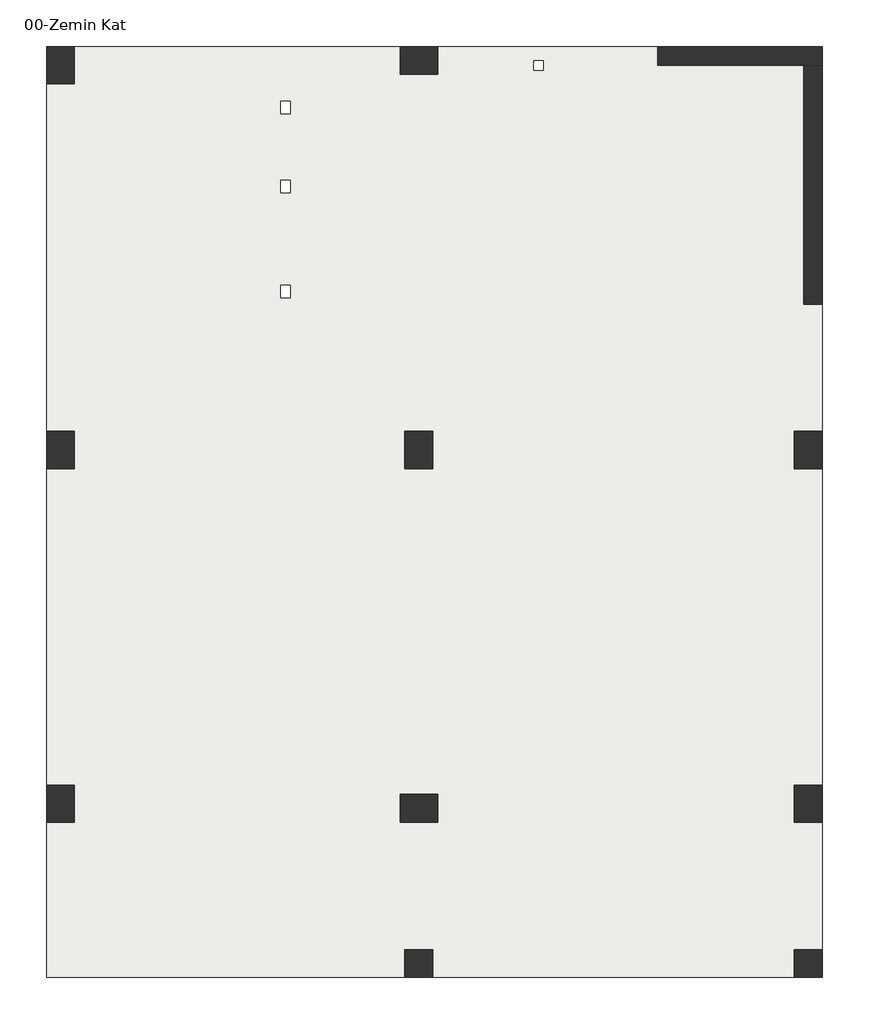
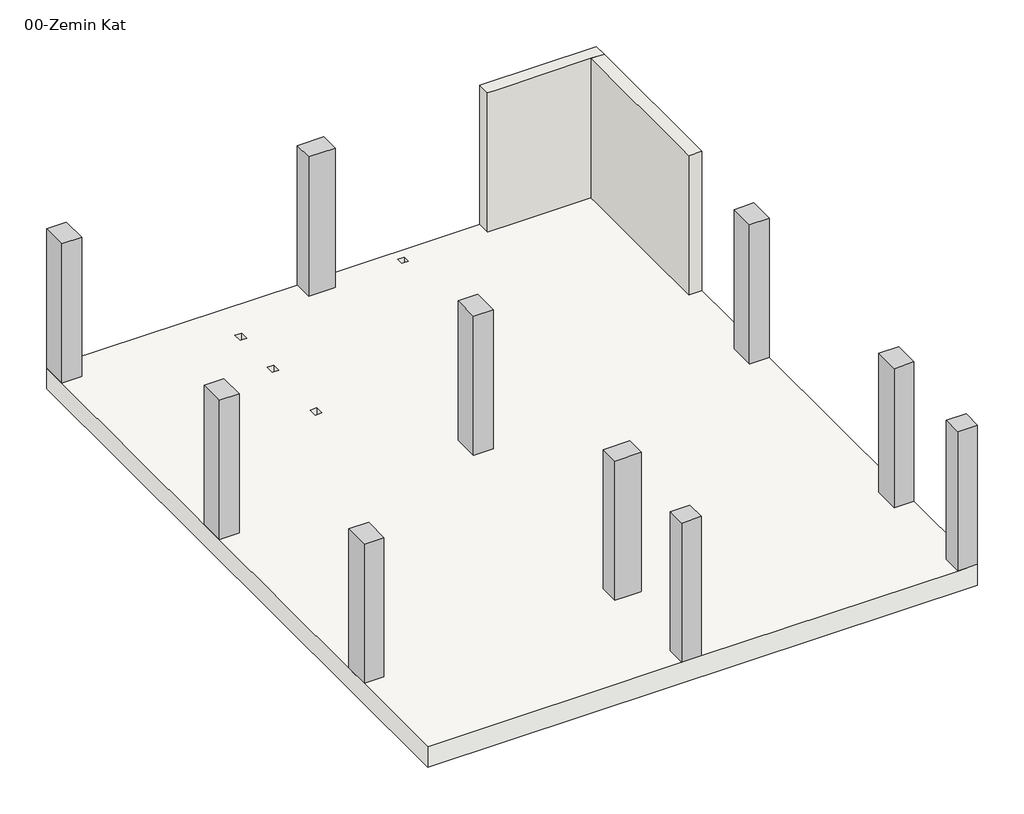
# One storey: 10 columns, 2 walls, 1 slab.
"""IFC4 building model written with IfcOpenShell, lengths in millimetres."""

from ifc_helpers import new_model, si_unit, frame, origin, place, context, project, spatial, polyline, outline, extrude, faceted_brep, element, save

model = new_model("IFC4")

# Units and contexts
model_context = context("Model", 3, world=origin())
ifc_project = project(units=[si_unit("LENGTHUNIT", "METRE", prefix="MILLI")], contexts=[model_context])

# Site, building, storey
site = spatial("IfcSite", under=ifc_project)
building = spatial("IfcBuilding", under=site)
storey = spatial("IfcBuildingStorey", under=building, Name="00-Zemin Kat", Elevation=93780.0)

# Columns
placement = place(None, origin())
element("IfcColumn", 1, ObjectType="M_Concrete-Rectangular-Column : 45x60cm Kolon", at=placement, inside=storey, context=model_context, shape_type="SweptSolid", body=[
    extrude(outline(polyline([(450.0, 15000.0), (450.0, 14400.0), (0.0, 14400.0), (0.0, 15000.0), (450.0, 15000.0)])), frame((0.0, 0.0, 93780.0), z_axis=(0.0, 0.0, 1.0), x_axis=(1.0, 0.0, 0.0)), (0.0, 0.0, 1.0), 3350.0),
])
element("IfcColumn", 2, ObjectType="M_Concrete-Rectangular-Column : 45x60cm Kolon", at=placement, inside=storey, context=model_context, shape_type="SweptSolid", body=[
    extrude(outline(polyline([(450.0, 8800.0), (450.0, 8200.0), (0.0, 8200.0), (0.0, 8800.0), (450.0, 8800.0)])), frame((0.0, 0.0, 93780.0), z_axis=(0.0, 0.0, 1.0), x_axis=(1.0, 0.0, 0.0)), (0.0, 0.0, 1.0), 3350.0),
])
element("IfcColumn", 3, ObjectType="M_Concrete-Rectangular-Column : 45x60cm Kolon", at=placement, inside=storey, context=model_context, shape_type="SweptSolid", body=[
    extrude(outline(polyline([(450.0, 3100.0), (450.0, 2500.0), (0.0, 2500.0), (0.0, 3100.0), (450.0, 3100.0)])), frame((0.0, 0.0, 93780.0), z_axis=(0.0, 0.0, 1.0), x_axis=(1.0, 0.0, 0.0)), (0.0, 0.0, 1.0), 3350.0),
])
element("IfcColumn", 4, ObjectType="M_Concrete-Rectangular-Column : 45x60cm Kolon", at=placement, inside=storey, context=model_context, shape_type="SweptSolid", body=[
    extrude(outline(polyline([(6225.0, 8800.0), (6225.0, 8200.0), (5775.0, 8200.0), (5775.0, 8800.0), (6225.0, 8800.0)])), frame((0.0, 0.0, 93780.0), z_axis=(0.0, 0.0, 1.0), x_axis=(1.0, 0.0, 0.0)), (0.0, 0.0, 1.0), 3350.0),
])
element("IfcColumn", 5, ObjectType="M_Concrete-Rectangular-Column : 45x60cm Kolon", at=placement, inside=storey, context=model_context, shape_type="SweptSolid", body=[
    extrude(outline(polyline([(12500.0, 8800.0), (12500.0, 8200.0), (12050.0, 8200.0), (12050.0, 8800.0), (12500.0, 8800.0)])), frame((0.0, 0.0, 93780.0), z_axis=(0.0, 0.0, 1.0), x_axis=(1.0, 0.0, 0.0)), (0.0, 0.0, 1.0), 3350.0),
])
element("IfcColumn", 6, ObjectType="M_Concrete-Rectangular-Column : 45x60cm Kolon", at=placement, inside=storey, context=model_context, shape_type="SweptSolid", body=[
    extrude(outline(polyline([(12500.0, 3100.0), (12500.0, 2500.0), (12050.0, 2500.0), (12050.0, 3100.0), (12500.0, 3100.0)])), frame((0.0, 0.0, 93780.0), z_axis=(0.0, 0.0, 1.0), x_axis=(1.0, 0.0, 0.0)), (0.0, 0.0, 1.0), 3350.0),
])
element("IfcColumn", 7, ObjectType="M_Concrete-Rectangular-Column : 45x60cm Kolon", at=placement, inside=storey, context=model_context, shape_type="SweptSolid", body=[
    extrude(outline(polyline([(5700.0, 15000.0), (6300.0, 15000.0), (6300.0, 14550.0), (5700.0, 14550.0), (5700.0, 15000.0)])), frame((0.0, 0.0, 93780.0), z_axis=(0.0, 0.0, 1.0), x_axis=(1.0, 0.0, 0.0)), (0.0, 0.0, 1.0), 3350.0),
])
element("IfcColumn", 8, ObjectType="M_Concrete-Rectangular-Column : 45x45cm Kolon", at=placement, inside=storey, context=model_context, shape_type="SweptSolid", body=[
    extrude(outline(polyline([(6225.0, 450.0), (6225.0, 0.0), (5775.0, 0.0), (5775.0, 450.0), (6225.0, 450.0)])), frame((0.0, 0.0, 93780.0), z_axis=(0.0, 0.0, 1.0), x_axis=(1.0, 0.0, 0.0)), (0.0, 0.0, 1.0), 3350.0),
])
element("IfcColumn", 9, ObjectType="M_Concrete-Rectangular-Column : 45x60cm Kolon", at=placement, inside=storey, context=model_context, shape_type="SweptSolid", body=[
    extrude(outline(polyline([(5700.0, 2950.0), (6300.0, 2950.0), (6300.0, 2500.0), (5700.0, 2500.0), (5700.0, 2950.0)])), frame((0.0, 0.0, 93780.0), z_axis=(0.0, 0.0, 1.0), x_axis=(1.0, 0.0, 0.0)), (0.0, 0.0, 1.0), 3350.0),
])
element("IfcColumn", 10, ObjectType="M_Concrete-Rectangular-Column : 45x45cm Kolon", at=placement, inside=storey, context=model_context, shape_type="SweptSolid", body=[
    extrude(outline(polyline([(12500.0, 450.0), (12500.0, 0.0), (12050.0, 0.0), (12050.0, 450.0), (12500.0, 450.0)])), frame((0.0, 0.0, 93780.0), z_axis=(0.0, 0.0, 1.0), x_axis=(1.0, 0.0, 0.0)), (0.0, 0.0, 1.0), 3350.0),
])

# Slab
element("IfcSlab", 11, ObjectType="50 cm döşeme", at=placement, inside=storey, context=model_context, shape_type="Brep", body=[
    faceted_brep([(12500.0, 15000.0, 93280.0), (12500.0, 0.0, 93280.0), (0.0, 0.0, 93280.0), (0.0, 15000.0, 93280.0), (3925.0, 14120.0, 93280.0), (3775.0, 14120.0, 93280.0), (3775.0, 13920.0, 93280.0), (3925.0, 13920.0, 93280.0), (3925.0, 12846.5789726, 93280.0), (3775.0, 12846.5789726, 93280.0), (3775.0, 12646.5789726, 93280.0), (3925.0, 12646.5789726, 93280.0), (3925.0, 11154.975, 93280.0), (3775.0, 11154.975, 93280.0), (3775.0, 10954.975, 93280.0), (3925.0, 10954.975, 93280.0), (7852.5, 14620.0, 93280.0), (8002.5, 14620.0, 93280.0), (8002.5, 14770.0, 93280.0), (7852.5, 14770.0, 93280.0), (12500.0, 15000.0, 93780.0), (6300.0, 15000.0, 93780.0), (5700.0, 15000.0, 93780.0), (450.0, 15000.0, 93780.0), (0.0, 15000.0, 93780.0), (0.0, 14400.0, 93780.0), (0.0, 8800.0, 93780.0), (0.0, 8200.0, 93780.0), (0.0, 3100.0, 93780.0), (0.0, 2500.0, 93780.0), (0.0, 0.0, 93780.0), (5775.0, 0.0, 93780.0), (6225.0, 0.0, 93780.0), (12050.0, 0.0, 93780.0), (12500.0, 0.0, 93780.0), (12500.0, 450.0, 93780.0), (12500.0, 2500.0, 93780.0), (12500.0, 3100.0, 93780.0), (12500.0, 8200.0, 93780.0), (12500.0, 8800.0, 93780.0), (3925.0, 14120.0, 93780.0), (3925.0, 13920.0, 93780.0), (3775.0, 13920.0, 93780.0), (3775.0, 14120.0, 93780.0), (3925.0, 12846.5789726, 93780.0), (3925.0, 12646.5789726, 93780.0), (3775.0, 12646.5789726, 93780.0), (3775.0, 12846.5789726, 93780.0), (3925.0, 11154.975, 93780.0), (3925.0, 10954.975, 93780.0), (3775.0, 10954.975, 93780.0), (3775.0, 11154.975, 93780.0), (7852.5, 14620.0, 93780.0), (7852.5, 14770.0, 93780.0), (8002.5, 14770.0, 93780.0), (8002.5, 14620.0, 93780.0)], [[[0, 1, 2, 3], [4, 5, 6, 7], [8, 9, 10, 11], [12, 13, 14, 15], [16, 17, 18, 19]], [[20, 21, 22, 23, 24, 25, 26, 27, 28, 29, 30, 31, 32, 33, 34, 35, 36, 37, 38, 39], [40, 41, 42, 43], [44, 45, 46, 47], [48, 49, 50, 51], [52, 53, 54, 55]], [[1, 0, 20, 39, 38, 37, 36, 35, 34]], [[2, 1, 34, 33, 32, 31, 30]], [[3, 2, 30, 29, 28, 27, 26, 25, 24]], [[0, 3, 24, 23, 22, 21, 20]], [[5, 4, 40, 43]], [[6, 5, 43, 42]], [[7, 6, 42, 41]], [[4, 7, 41, 40]], [[9, 8, 44, 47]], [[10, 9, 47, 46]], [[11, 10, 46, 45]], [[8, 11, 45, 44]], [[13, 12, 48, 51]], [[14, 13, 51, 50]], [[15, 14, 50, 49]], [[12, 15, 49, 48]], [[17, 16, 52, 55]], [[18, 17, 55, 54]], [[19, 18, 54, 53]], [[16, 19, 53, 52]]]),
])

# Walls
element("IfcWall", 12, ObjectType="30cm Perde Duvar", at=placement, inside=storey, context=model_context, shape_type="Brep", body=[
    faceted_brep([(9850.0, 14700.0, 93780.0), (12200.0, 14700.0, 93780.0), (12500.0, 14700.0, 93780.0), (12500.0, 14700.0, 97130.0), (12200.0, 14700.0, 97130.0), (10000.0, 14700.0, 97130.0), (9850.0, 14700.0, 97130.0), (9850.0, 14700.0, 96680.0), (9850.0, 15000.0, 93780.0), (9850.0, 15000.0, 96680.0), (9850.0, 15000.0, 97130.0), (12500.0, 15000.0, 97130.0), (12500.0, 15000.0, 93780.0)], [[[0, 1, 2, 3, 4, 5, 6, 7]], [[8, 9, 10, 11, 12]], [[2, 1, 0, 8, 12]], [[0, 7, 6, 10, 9, 8]], [[3, 2, 12, 11]], [[6, 5, 4, 3, 11, 10]]]),
])
element("IfcWall", 13, ObjectType="30cm Perde Duvar", at=placement, inside=storey, context=model_context, shape_type="Brep", body=[
    faceted_brep([(12200.0, 14700.0, 93780.0), (12200.0, 10850.0, 93780.0), (12200.0, 10850.0, 96680.0), (12200.0, 10850.0, 97130.0), (12200.0, 11000.0, 97130.0), (12200.0, 14700.0, 97130.0), (12500.0, 14700.0, 93780.0), (12500.0, 14700.0, 97130.0), (12500.0, 10850.0, 97130.0), (12500.0, 10850.0, 96680.0), (12500.0, 10850.0, 93780.0)], [[[0, 1, 2, 3, 4, 5]], [[6, 7, 8, 9, 10]], [[1, 0, 6, 10]], [[3, 2, 1, 10, 9, 8]], [[0, 5, 7, 6]], [[5, 4, 3, 8, 7]]]),
])

save(model, "model.ifc")

# Revit data of these elements
# Project information
#   Project Issue Date = "Issue Date"
#   Project Status = "Project Status"
#   Client Name = "Owner"
#   Project Address = "Enter address here"
#   Project Name = "Project Name"
#   Project Number = "0001"
# Grids (mm)
#   "1": line (0, -1446.356) -> (0, 16597.874)
#   "2": line (6000, -1446.356) -> (6000, 16597.874)
#   "3": line (12500, -1446.356) -> (12500, 16597.874)
#   "A": line (-3259.789, 0) -> (14827.9, 0)
#   "B": line (-3259.789, 2500) -> (14827.9, 2500)
#   "C": line (-3259.789, 8500) -> (14827.9, 8500)
#   "D": line (-3259.789, 15000) -> (14827.9, 15000)
# Type "M_Concrete-Rectangular-Column : 45x60cm Kolon"
#   b = 45.00 cm
#   h = 60.00 cm
#   Structural Material [instance default] = Concrete, Cast-in-Place gray
# Type "M_Concrete-Rectangular-Column : 45x45cm Kolon"
#   b = 45.00 cm
#   h = 45.00 cm
#   Structural Material [instance default] = Concrete, Cast-in-Place gray
# Type "50 cm döşeme"
#   Function = 0
#   Layers, outside or top first: 50.00 cm "Concrete, Cast In Situ" (function 1)
# Type "30cm Perde Duvar"
#   Layers, outside or top first: 30.00 cm "Concrete, Cast In Situ" (function 1)
# Elements 1, 2, 3, 4, 5, 6, 7, 9 (IfcColumn, "M_Concrete-Rectangular-Column : 45x60cm Kolon")
#   Comments = ""
#   Structural Material = Concrete, Cast-in-Place gray
#   Phase Created = New Construction
#   Materials on its faces: "Concrete, Cast-in-Place gray"
# Elements 8, 10 (IfcColumn, "M_Concrete-Rectangular-Column : 45x45cm Kolon")
#   Comments = ""
#   Structural Material = Concrete, Cast-in-Place gray
#   Phase Created = New Construction
#   Materials on its faces: "Concrete, Cast-in-Place gray"
# Element 11 (IfcSlab, "50 cm döşeme")
#   Height Offset From Level = 0.00 cm
#   built-in parameter 1001954 = 1
#   Phase Created = New Construction
#   Materials on its faces: "Concrete, Cast In Situ"
# Elements 12, 13 (IfcWall, "30cm Perde Duvar")
#   Comments = ""
#   Top Offset = 0.00 cm
#   Base Offset = 0.00 cm
#   wall height = 335.00 cm
#   Phase Created = New Construction
#   Base Constraint = 00-Zemin Kat
#   Top Constraint = 01-Birinci Kat
#   Materials on its faces: "Concrete, Cast In Situ"
# Materials
#   "Concrete, Cast-in-Place gray": class "Concrete", colour RGB 192 192 192, transparency 0, Description = "Cast-in-place concrete", Cost = 0
#   "Concrete, Cast In Situ": class "Concrete", colour RGB 192 192 192, transparency 0, Description = "physical material", Cost = 0
